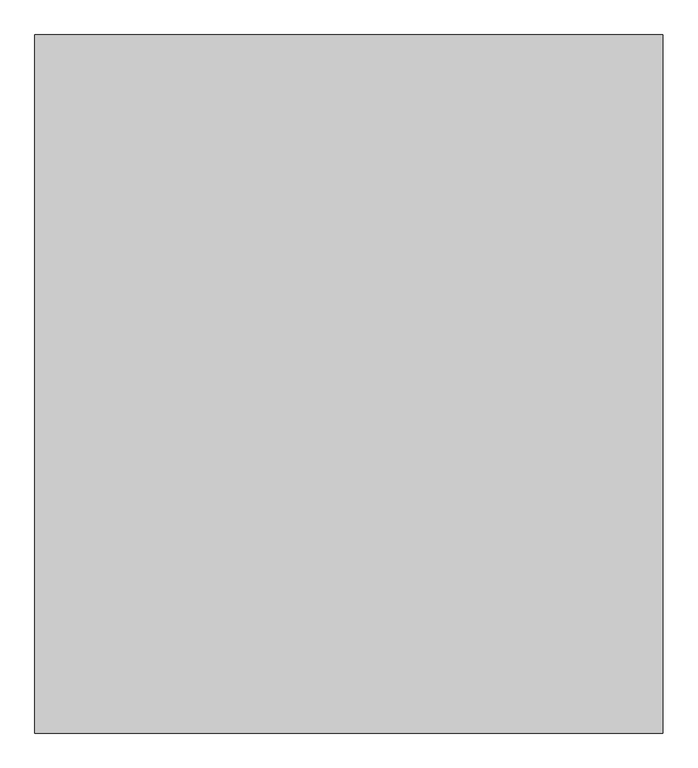
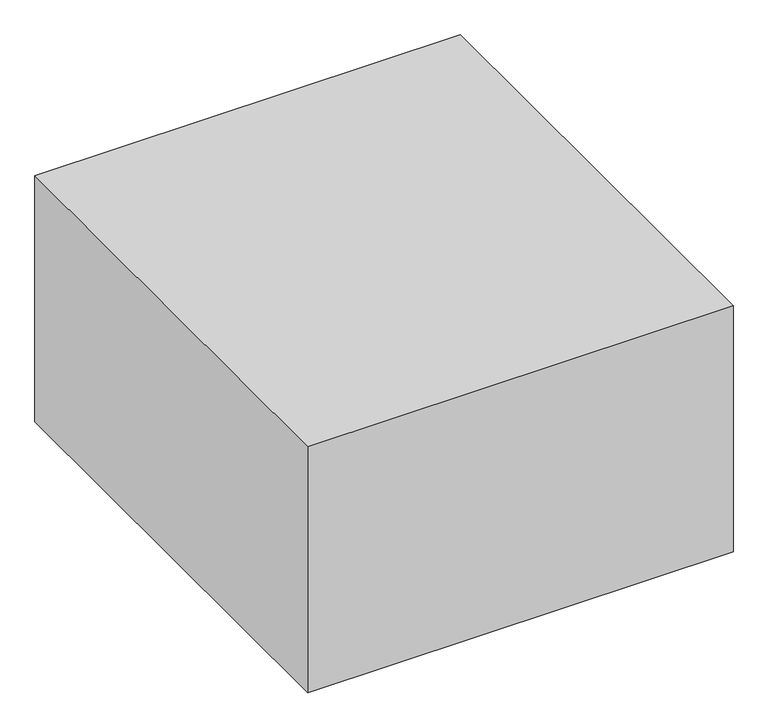
"""IFC4 building model written with IfcOpenShell, lengths in millimetres: proxy geometry, Space Planning Box_hec : Space Planning Box_hec."""

import ifcopenshell
import ifcopenshell.guid

model = None  # the IFC model being written
_history = None  # IfcOwnerHistory: only IFC2X3 demands one
_inside = {}  # id of a spatial element -> (the spatial element, [elements in it])
_under = {}  # id of a project, library or spatial element -> (it, [spatial elements below it])
_declared = {}  # id of a project -> (the project, [libraries it declares])
_typed = {}  # id of a type object -> (the type object, [elements of that type])
_made_of = {}  # id of a material, layer set ... -> (it, [elements and type objects made of it])


def new_model(schema):
    """Start an empty IFC model of exactly this schema.

    Asked for "IFC4X3", IfcOpenShell would pick the latest addendum, in which some entities
    have other attributes; the version numbers below select the first issue.
    IFC2X3 requires an IfcOwnerHistory on every rooted entity: one is made here for all.
    """
    global model, _history
    if schema == "IFC4X3":
        model = ifcopenshell.file(schema_version=(4, 3, 0, 0))
    else:
        model = ifcopenshell.file(schema=schema)
    _inside.clear()
    _under.clear()
    _declared.clear()
    _typed.clear()
    _made_of.clear()
    _history = None
    if model.schema == "IFC2X3":
        org = make("IfcOrganization", Name="unknown")
        user = make(
            "IfcPersonAndOrganization",
            ThePerson=make("IfcPerson", FamilyName="unknown"),
            TheOrganization=org,
        )
        app = make(
            "IfcApplication",
            ApplicationDeveloper=org,
            Version="unknown",
            ApplicationFullName="unknown",
            ApplicationIdentifier="unknown",
        )
        _history = make(
            "IfcOwnerHistory",
            OwningUser=user,
            OwningApplication=app,
            ChangeAction="ADDED",
            CreationDate=0,
        )
    return model


def make(cls, **values):
    """One entity of the class cls with the attributes given. An attribute that is None is left unset."""
    return model.create_entity(
        cls, **{name: value for name, value in values.items() if value is not None}
    )


def rooted(cls, **values):
    """An entity with a GlobalId (a new one), such as an element, a storey or a relation."""
    return make(cls, GlobalId=ifcopenshell.guid.new(), OwnerHistory=_history, **values)


def si_unit(unit_type, name, prefix=None):
    """IfcSIUnit, for example si_unit("LENGTHUNIT", "METRE", prefix="MILLI")."""
    return make("IfcSIUnit", UnitType=unit_type, Prefix=prefix, Name=name)


def assignment(units):
    """IfcUnitAssignment: the units of a project."""
    return None if units is None else make("IfcUnitAssignment", Units=units)


def point(xyz):
    """IfcCartesianPoint."""
    return None if xyz is None else make("IfcCartesianPoint", Coordinates=xyz)


def direction(xyz):
    """IfcDirection."""
    return None if xyz is None else make("IfcDirection", DirectionRatios=xyz)


def frame(location, z_axis=None, x_axis=None):
    """IfcAxis2Placement3D, a coordinate frame: its origin and axes. An axis left out is left unset."""
    return make(
        "IfcAxis2Placement3D",
        Location=point(location),
        Axis=direction(z_axis),
        RefDirection=direction(x_axis),
    )


def origin():
    """The frame at (0, 0, 0) with its axes left unset."""
    return frame((0.0, 0.0, 0.0))


def origin_with_axes():
    """The frame at (0, 0, 0) with the z axis (0, 0, 1) and the x axis (1, 0, 0) written out."""
    return frame((0.0, 0.0, 0.0), z_axis=(0.0, 0.0, 1.0), x_axis=(1.0, 0.0, 0.0))


def place(relative_to, where):
    """IfcLocalPlacement: puts the frame where relative to a parent placement (None: the world)."""
    return make(
        "IfcLocalPlacement", PlacementRelTo=relative_to, RelativePlacement=where
    )


def context(
    kind, dimensions, precision=None, world=None, true_north=None, identifier=None
):
    """IfcGeometricRepresentationContext, for example the 3D "Model" context."""
    return make(
        "IfcGeometricRepresentationContext",
        ContextIdentifier=identifier,
        ContextType=kind,
        CoordinateSpaceDimension=dimensions,
        Precision=precision,
        WorldCoordinateSystem=world,
        TrueNorth=true_north,
    )


def project(units=None, contexts=None):
    """IfcProject with its units and contexts."""
    return rooted(
        "IfcProject",
        Name="project",
        RepresentationContexts=contexts,
        UnitsInContext=assignment(units),
    )


def spatial(cls, under=None, at=None, **own):
    """A site, building, storey or space (cls), placed at a placement, below another one or the project."""
    s = rooted(cls, ObjectPlacement=at, **own)
    if under is not None:
        _under.setdefault(under.id(), (under, []))[1].append(s)
    return s


def polyline(points):
    """IfcPolyline through the points."""
    return make("IfcPolyline", Points=[point(p) for p in points])


def outline(outer, holes=None, kind="AREA"):
    """IfcArbitraryClosedProfileDef: a profile drawn as a closed curve; with holes, ...WithVoids."""
    if holes is None:
        return make("IfcArbitraryClosedProfileDef", ProfileType=kind, OuterCurve=outer)
    return make(
        "IfcArbitraryProfileDefWithVoids",
        ProfileType=kind,
        OuterCurve=outer,
        InnerCurves=holes,
    )


def extrude(swept, where, along, depth):
    """IfcExtrudedAreaSolid: the profile swept, set in the frame where, extruded along a direction by depth."""
    return make(
        "IfcExtrudedAreaSolid",
        SweptArea=swept,
        Position=where,
        ExtrudedDirection=direction(along),
        Depth=depth,
    )


def shape(context_of_items, identifier, shape_type, items):
    """IfcShapeRepresentation: the items that make up one representation, for example the "Body"."""
    return make(
        "IfcShapeRepresentation",
        ContextOfItems=context_of_items,
        RepresentationIdentifier=identifier,
        RepresentationType=shape_type,
        Items=items,
    )


def source(mapping_origin, context_of_items, identifier, shape_type, items):
    """IfcRepresentationMap: a shape defined once, which mapped items show again and again."""
    return make(
        "IfcRepresentationMap",
        MappingOrigin=mapping_origin,
        MappedRepresentation=shape(context_of_items, identifier, shape_type, items),
    )


def transform(
    local_origin,
    x_axis=None,
    y_axis=None,
    z_axis=None,
    scale=None,
    scale2=None,
    scale3=None,
    uniform=True,
):
    """IfcCartesianTransformationOperator3D, or its non-uniform kind. x_axis, y_axis, z_axis: its Axis1, 2, 3."""
    if uniform:
        return make(
            "IfcCartesianTransformationOperator3D",
            Axis1=direction(x_axis),
            Axis2=direction(y_axis),
            LocalOrigin=point(local_origin),
            Scale=scale,
            Axis3=direction(z_axis),
        )
    return make(
        "IfcCartesianTransformationOperator3DnonUniform",
        Axis1=direction(x_axis),
        Axis2=direction(y_axis),
        LocalOrigin=point(local_origin),
        Scale=scale,
        Axis3=direction(z_axis),
        Scale2=scale2,
        Scale3=scale3,
    )


def mapped(mapping_source, mapping_target):
    """IfcMappedItem: shows the shape of a source again, moved by a transform."""
    return make(
        "IfcMappedItem", MappingSource=mapping_source, MappingTarget=mapping_target
    )


def made_of(thing, what):
    """Note that an element or type object is made of a material, layer set ...; save() writes the relation."""
    if what is not None:
        _made_of.setdefault(what.id(), (what, []))[1].append(thing)
    return thing


def element(
    cls,
    number,
    at=None,
    inside=None,
    cuts=None,
    type_object=None,
    material=None,
    context=None,
    identifier="Body",
    shape_type=None,
    held_by="IfcProductDefinitionShape",
    body=None,
    shapes=None,
    **own,
):
    """One element of the class cls, such as IfcWall. Its Tag is "e" and its number.

    at: its placement. inside: the storey or other place that contains it. cuts: it is an
    opening in that element (IfcRelVoidsElement). A single representation is given by context,
    identifier, shape_type and body (its items); several are given by shapes. held_by: the class
    of the entity that holds the representations. save() writes the other relations.
    """
    e = rooted(cls, Tag="e%d" % number, ObjectPlacement=at, **own)
    if body is not None:
        shapes = [shape(context, identifier, shape_type, body)]
    if shapes is not None:
        e.Representation = make(held_by, Representations=shapes)
    if inside is not None:
        _inside.setdefault(inside.id(), (inside, []))[1].append(e)
    if cuts is not None:
        rooted(
            "IfcRelVoidsElement", RelatingBuildingElement=cuts, RelatedOpeningElement=e
        )
    if type_object is not None:
        _typed.setdefault(type_object.id(), (type_object, []))[1].append(e)
    return made_of(e, material)


def aggregate(whole, parts):
    """IfcRelAggregates: a whole, such as a stair, and the parts it consists of."""
    return rooted("IfcRelAggregates", RelatingObject=whole, RelatedObjects=parts)


def save(model, path):
    """Write the relations noted so far, then the file.

    IfcRelAggregates (storeys below a building ...), IfcRelContainedInSpatialStructure (elements
    in a storey), IfcRelDefinesByType, IfcRelAssociatesMaterial and IfcRelDeclares: one each for
    every whole, place, type object, material and project.
    """
    for whole, parts in _under.values():
        aggregate(whole, parts)
    for where, things in _inside.values():
        rooted(
            "IfcRelContainedInSpatialStructure",
            RelatedElements=things,
            RelatingStructure=where,
        )
    for kind, things in _typed.values():
        rooted("IfcRelDefinesByType", RelatedObjects=things, RelatingType=kind)
    for what, things in _made_of.values():
        rooted("IfcRelAssociatesMaterial", RelatedObjects=things, RelatingMaterial=what)
    for by, libraries in _declared.values():
        rooted("IfcRelDeclares", RelatingContext=by, RelatedDefinitions=libraries)
    model.write(path)


def generic_models_2d265e4a(model_context):
    return source(origin(), model_context, "Body", "SweptSolid", [
        extrude(outline(polyline([(4500.0, 5000.0), (4500.0, -5000.0), (-4500.0, -5000.0), (-4500.0, 5000.0), (4500.0, 5000.0)])), origin_with_axes(), (0.0, 0.0, 1.0), 5500.0),
    ])


if __name__ == "__main__":
    model = new_model("IFC4")
    model_context = context("Model", 3, world=origin())
    ifc_project = project(units=[si_unit("LENGTHUNIT", "METRE", prefix="MILLI")], contexts=[model_context])
    site = spatial("IfcSite", under=ifc_project)
    building = spatial("IfcBuilding", under=site)
    placement = place(None, origin())
    generic_models_shape = generic_models_2d265e4a(model_context)
    element("IfcBuildingElementProxy", 1, Name="Space Planning Box_hec : Space Planning Box_hec", ObjectType="Space Planning Box_hec : Space Planning Box_hec", at=placement, inside=building, context=model_context, shape_type="MappedRepresentation", body=[
        mapped(generic_models_shape, transform((0.0, 0.0, 0.0), x_axis=(1.0, 0.0, 0.0), y_axis=(0.0, 1.0, 0.0), z_axis=(0.0, 0.0, 1.0))),
    ])
    save(model, "model.ifc")

# Revit data of these elements
# Type "Space Planning Box_hec : Space Planning Box_hec"
#   Type Comments = "..."
#   Room Name [instance default] = "?"
#   Interior Finish [instance default] = ""
#   Exterior Finish [instance default] = ""
#   Department [instance default] = ""
#   Assembly Code = "..."
#   ceiling height [instance default] = 0
#   Width [instance default] = 1524 mm
#   Program Area [instance default] = 0.00 m²
#   Length [instance default] = 1524 mm
#   Height [instance default] = 1524 mm
#   Area [instance default] = 2.32258 m²
#   Fill Color [instance default] = Cyan
#   Default Elevation = 0
# Element 1 (IfcBuildingElementProxy, "Space Planning Box_hec : Space Planning Box_hec")
#   Room Name = "Electrical Room (GIS)"
#   Exterior Finish = "N/A..N/A,,EW1..EW2..N/A"
#   Department = "AR"
#   Width = 9000 mm
#   Program Area = 90.00 m²
#   Length = 10000 mm
#   Height = 5500 mm
#   Area = 90.00 m²
#   Materials on its faces: "Cyan"
# Materials
#   "Cyan": class "Generic", colour RGB 0 255 255, transparency 0.2, Cost = 0
